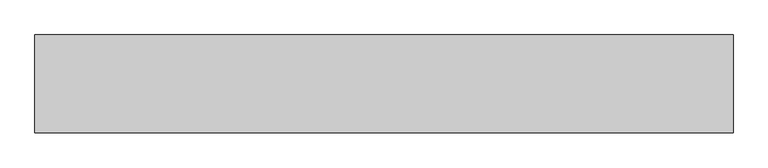
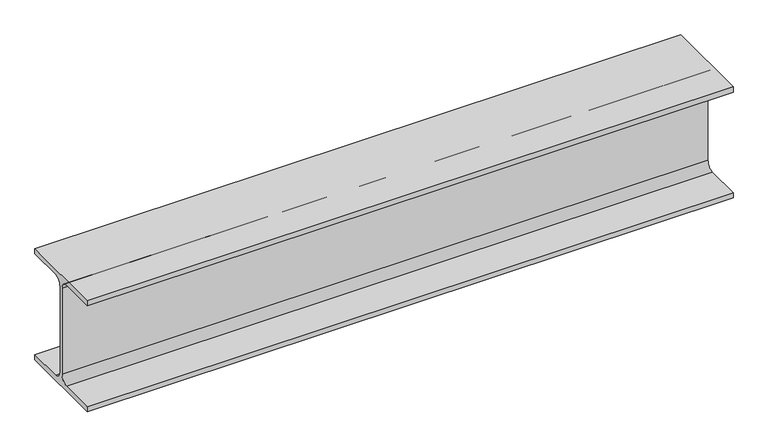
"""IFC4 building model written with IfcOpenShell, lengths in millimetres: beam geometry, 0912_Steel Framing_H-KSD3502 : H_SB_ASB_H-194x150x6x9."""

from ifc_helpers import new_model, si_unit, point, frame, frame_2d, origin, place, context, project, spatial, polyline, circle_curve, trimmed, segment, composite_curve, outline, extrude, source, transform, mapped, element, save


def beam_70886e5f(model_context):
    return source(origin(), model_context, "Body", "SweptSolid", [
        extrude(outline(composite_curve([segment(polyline([(-75.0, -88.0), (-16.0, -88.0)]), True, "CONTINUOUS"), segment(trimmed(circle_curve(frame_2d((-16.0, -75.0)), 13.0), [point((-16.0, -88.0))], [point((-3.0, -75.0))], True, "CARTESIAN"), True, "CONTINUOUS"), segment(polyline([(-3.0, -75.0), (-3.0, 75.0)]), True, "CONTINUOUS"), segment(trimmed(circle_curve(frame_2d((-16.0, 75.0)), 13.0), [point((-3.0, 75.0))], [point((-16.0, 88.0))], True, "CARTESIAN"), True, "CONTINUOUS"), segment(polyline([(-16.0, 88.0), (-75.0, 88.0), (-75.0, 97.0), (75.0, 97.0), (75.0, 88.0), (16.0, 88.0)]), True, "CONTINUOUS"), segment(trimmed(circle_curve(frame_2d((16.0, 75.0)), 13.0), [point((16.0, 88.0))], [point((3.0, 75.0))], True, "CARTESIAN"), True, "CONTINUOUS"), segment(polyline([(3.0, 75.0), (3.0, -75.0)]), True, "CONTINUOUS"), segment(trimmed(circle_curve(frame_2d((16.0, -75.0)), 13.0), [point((3.0, -75.0))], [point((16.0, -88.0))], True, "CARTESIAN"), True, "CONTINUOUS"), segment(polyline([(16.0, -88.0), (75.0, -88.0), (75.0, -97.0), (-75.0, -97.0), (-75.0, -88.0)]), True, "CONTINUOUS")], self_intersect=False)), frame((-293.5180628, 0.0, 0.0), z_axis=(1.0, 0.0, 0.0), x_axis=(0.0, 1.0, 0.0)), (0.0, 0.0, 1.0), 1068.0320464),
    ])


if __name__ == "__main__":
    model = new_model("IFC4")
    model_context = context("Model", 3, world=origin())
    ifc_project = project(units=[si_unit("LENGTHUNIT", "METRE", prefix="MILLI")], contexts=[model_context])
    site = spatial("IfcSite", under=ifc_project)
    building = spatial("IfcBuilding", under=site)
    placement = place(None, origin())
    beam_shape = beam_70886e5f(model_context)
    element("IfcBeam", 1, ObjectType="0912_Steel Framing_H-KSD3502 : H_SB_ASB_H-194x150x6x9", at=placement, inside=building, context=model_context, shape_type="MappedRepresentation", body=[
        mapped(beam_shape, transform((0.0, 0.0, 0.0), x_axis=(1.0, 0.0, 0.0), y_axis=(0.0, 1.0, 0.0), z_axis=(0.0, 0.0, 1.0))),
    ])
    save(model, "model.ifc")

# Revit data of these elements
# Type "0912_Steel Framing_H-KSD3502 : H_SB_ASB_H-194x150x6x9"
#   H_WM Code_1 = "S01AA002-00001 | Main Steel Structure Fabrication Work | Shelter/Building | Medium Steel - Standard (90KG/M>Weight≥30KG/M) | Material: (   )"
#   H_WM Code_2 = "S03AA028-00001 | Main Steel Structure Erection Work | Shelter/Building | Medium Steel (90KG/M>Weight≥30KG/M) | Material: (   )"
#   H_WM Code_3 = "S01AA010-00001 | Main Steel Structure Fabrication Work | Shelter/Building | Steel Painting/Coating | for Non-Fireproofed Steel Surface, Surface Preparation, Primer, Second & Final Coat | Material: (   )"
#   H_Q'ty Cal Type Tag = "SB-Q2"
#   Width = 15.0 cm
#   Web Thickness = 0.6 cm
#   Web Fillet = 1.3 cm
#   Warping Constant = 43316.0 cm⁶
#   W = 0
#   Torsional Moment of Inertia = 8.622 cm⁴
#   Section Area = 39.01 cm²
#   Plastic Modulus weak axis = 104.0 cm³
#   Plastic Modulus strong axis = 309.0 cm³
#   Perimeter = 0.95 m²/m
#   Nominal Weight = 30.60 kgf/m
#   Moment of Inertia weak axis = 507.00 cm⁴
#   Moment of Inertia strong axis = 2690.00 cm⁴
#   Height = 19.4 cm
#   Flange Thickness = 0.9 cm
#   Elastic Modulus weak axis = 67.6 cm³
#   Elastic Modulus strong axis = 277.0 cm³
#   Centroid Vertical = 9.7 cm
#   Centroid Horizontal = 7.5 cm
#   Ix = 26900000
#   Length [instance default] = 1.5240 m
#   Zx = 309000
#   b = 0.1500 m
#   h = 0.1940 m
#   r = 0.0130 m
#   s = 0.0060 m
#   t = 0.0090 m
#   A = 0.003901 m²
#   Structural Material [instance default] = Steel, 45-345
#   Assembly Code = ""
# Element 1 (IfcBeam, "0912_Steel Framing_H-KSD3502 : H_SB_ASB_H-194x150x6x9")
#   Structural Material = none
# Materials
#   "Steel, 45-345": class "Metal", colour RGB 189 187 185, transparency 0, Description = "Steel 345 MPa", Cost = 0
